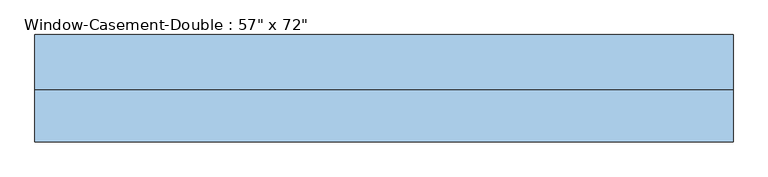
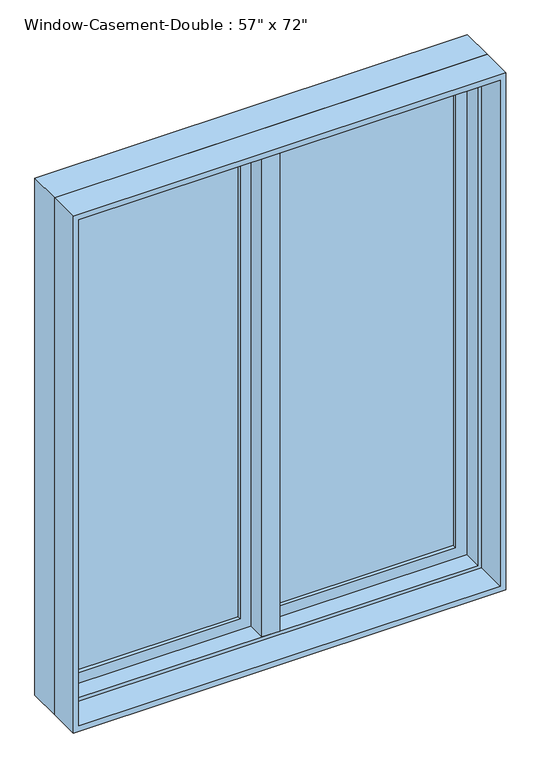
"""IFC4 building model written with IfcOpenShell, lengths in millimetres: window geometry."""

from ifc_helpers import new_model, si_unit, frame, origin, place, context, project, spatial, polyline, outline, extrude, faceted_brep, source, transform, mapped, element, save


def window_c580ef63(model_context):
    return source(origin(), model_context, "Body", "SolidModel", [
        faceted_brep([(9.525, 120.65, 2730.5), (-9.525, 120.65, 2730.5), (-9.525, 69.85, 2730.5), (9.525, 69.85, 2730.5), (9.525, 120.65, 927.1), (9.525, 69.85, 927.1), (-9.525, 69.85, 927.1), (-9.525, 120.65, 927.1), (-9.525, 69.85, 946.15), (-9.525, 69.85, 2711.45), (-30.1625, 69.85, 946.15), (-30.1625, 69.85, 2711.45), (-30.1625, 6.35, 946.15), (-30.1625, 6.35, 2711.45), (30.1625, 6.35, 946.15), (30.1625, 6.35, 2711.45), (30.1625, 69.85, 946.15), (30.1625, 69.85, 2711.45), (9.525, 69.85, 946.15), (9.525, 69.85, 2711.45)], [[[0, 1, 2, 3]], [[4, 5, 6, 7]], [[1, 0, 4, 7]], [[2, 1, 7, 6, 8, 9]], [[9, 8, 10, 11]], [[11, 10, 12, 13]], [[13, 12, 14, 15]], [[15, 14, 16, 17]], [[17, 16, 18, 19]], [[0, 3, 19, 18, 5, 4]], [[18, 8, 6, 5]], [[9, 19, 3, 2]], [[8, 18, 16, 14, 12, 10]], [[19, 9, 11, 13, 15, 17]]]),
        extrude(outline(polyline([(-66.675, 101.6), (-66.675, 95.25), (-654.05, 95.25), (-654.05, 101.6), (-66.675, 101.6)])), frame((0.0, 0.0, 984.25), z_axis=(0.0, 0.0, 1.0), x_axis=(1.0, 0.0, 0.0)), (0.0, 0.0, 1.0), 1689.1),
        extrude(outline(polyline([(-654.05, 82.55), (-654.05, 88.9), (-66.675, 88.9), (-66.675, 82.55), (-654.05, 82.55)])), frame((0.0, 0.0, 984.25), z_axis=(0.0, 0.0, 1.0), x_axis=(1.0, 0.0, 0.0)), (0.0, 0.0, 1.0), 1689.1),
        extrude(outline(polyline([(654.05, 101.6), (654.05, 95.25), (66.675, 95.25), (66.675, 101.6), (654.05, 101.6)])), frame((0.0, 0.0, 984.25), z_axis=(0.0, 0.0, 1.0), x_axis=(1.0, 0.0, 0.0)), (0.0, 0.0, 1.0), 1689.1),
        extrude(outline(polyline([(66.675, 82.55), (66.675, 88.9), (654.05, 88.9), (654.05, 82.55), (66.675, 82.55)])), frame((0.0, 0.0, 984.25), z_axis=(0.0, 0.0, 1.0), x_axis=(1.0, 0.0, 0.0)), (0.0, 0.0, 1.0), 1689.1),
        extrude(outline(polyline([(2730.5, -711.2), (927.1, -711.2), (927.1, -9.525), (2730.5, -9.525), (2730.5, -711.2)]), holes=[polyline([(2673.35, -66.675), (984.25, -66.675), (984.25, -654.05), (2673.35, -654.05), (2673.35, -66.675)])]), frame((0.0, 69.85, 0.0), z_axis=(0.0, 1.0, 0.0), x_axis=(0.0, 0.0, 1.0)), (0.0, 0.0, 1.0), 44.45),
        extrude(outline(polyline([(927.1, 711.2), (2730.5, 711.2), (2730.5, 9.525), (927.1, 9.525), (927.1, 711.2)]), holes=[polyline([(984.25, 66.675), (2673.35, 66.675), (2673.35, 654.05), (984.25, 654.05), (984.25, 66.675)])]), frame((0.0, 69.85, 0.0), z_axis=(0.0, 1.0, 0.0), x_axis=(0.0, 0.0, 1.0)), (0.0, 0.0, 1.0), 44.45),
        extrude(outline(polyline([(2743.2, -723.9), (914.4, -723.9), (914.4, 723.9), (2743.2, 723.9), (2743.2, -723.9)]), holes=[polyline([(2724.15, 704.85), (933.45, 704.85), (933.45, -704.85), (2724.15, -704.85), (2724.15, 704.85)])]), frame((0.0, -101.6, 0.0), z_axis=(0.0, 1.0, 0.0), x_axis=(0.0, 0.0, 1.0)), (0.0, 0.0, 1.0), 107.95),
        faceted_brep([(692.15, 69.85, 2711.45), (692.15, 6.35, 2711.45), (-692.15, 6.35, 2711.45), (-692.15, 69.85, 2711.45), (711.2, 120.65, 2730.5), (711.2, 69.85, 2730.5), (-711.2, 69.85, 2730.5), (-711.2, 120.65, 2730.5), (723.9, 6.35, 2743.2), (723.9, 120.65, 2743.2), (-723.9, 120.65, 2743.2), (-723.9, 6.35, 2743.2), (-692.15, 6.35, 946.15), (-692.15, 69.85, 946.15), (-711.2, 69.85, 927.1), (-711.2, 120.65, 927.1), (-723.9, 120.65, 914.4), (-723.9, 6.35, 914.4), (692.15, 6.35, 946.15), (692.15, 69.85, 946.15), (711.2, 69.85, 927.1), (711.2, 120.65, 927.1), (723.9, 120.65, 914.4), (723.9, 6.35, 914.4)], [[[0, 1, 2, 3]], [[4, 5, 6, 7]], [[8, 9, 10, 11]], [[3, 2, 12, 13]], [[7, 6, 14, 15]], [[11, 10, 16, 17]], [[13, 12, 18, 19]], [[15, 14, 20, 21]], [[17, 16, 22, 23]], [[11, 17, 23, 8], [1, 18, 12, 2]], [[19, 18, 1, 0]], [[5, 20, 14, 6], [3, 13, 19, 0]], [[21, 20, 5, 4]], [[23, 22, 9, 8]], [[9, 22, 16, 10], [7, 15, 21, 4]]]),
    ])


if __name__ == "__main__":
    model = new_model("IFC4")
    model_context = context("Model", 3, world=origin())
    ifc_project = project(units=[si_unit("LENGTHUNIT", "METRE", prefix="MILLI")], contexts=[model_context])
    site = spatial("IfcSite", under=ifc_project)
    building = spatial("IfcBuilding", under=site)
    placement = place(None, origin())
    window_shape = window_c580ef63(model_context)
    element("IfcWindow", 1, ObjectType="Window-Casement-Double : 57\" x 72\"", at=placement, inside=building, context=model_context, shape_type="MappedRepresentation", body=[
        mapped(window_shape, transform((0.0, 0.0, 0.0), x_axis=(1.0, 0.0, 0.0), y_axis=(0.0, 1.0, 0.0), z_axis=(0.0, 0.0, 1.0))),
    ])
    save(model, "model.ifc")

# Revit data of these elements
# Type "Window-Casement-Double : 57\" x 72\""
#   Type Mark = "62"
#   Fire Rating = "0.5h"
#   Assembly Code = "B2020100"
#   Analytic Construction = "Double glazing - domestic"
#   Frame Extension [instance default] = 0' - 0 1/4"
#   Window Inset [instance default] = 0' - 0"
#   Wall Thickness [instance default] = 0' - 6"
#   Interior Wall Closure [instance default] = 0' - 2 1/4"
#   Half Width = 2' - 4 1/2"
#   Visual Light Transmittance = 0.81
#   Thermal Resistance (R) = 1.8146 (h·ft²·°F)/BTU
#   Solar Heat Gain Coefficient = 0.76
#   Rough Width = 4' - 9 1/2"
#   Rough Height = 6' - 0 1/2"
#   Height = 6' - 0"
#   Heat Transfer Coefficient (U) = 0.5511 BTU/(h·ft²·°F)
#   Exterior Wall Closure [instance default] = 0' - 1 1/4"
#   Extension Jamb [instance default] = 0' - 2 1/4"
#   Default Sill Height = 3' - 0"
#   Width = 4' - 9"
#   Define Thermal Properties by = 0
#   Muntin Visibility = yes
#   Interior Trim Visibility [instance default] = yes
#   Exterior Trim Visibility [instance default] = yes
#   Extension Jamb Visibility [instance default] = yes
#   Interior Trim Material = Wood - Stained
#   Muntin Pattern = Muntin Pattern_2x2 : Muntin Pattern_2x2
#   Interior Trim = Trim-Window-Interior-Flat : Picture Frame
#   Interior Frame Material = Wood - Stained
#   Glass Panel Material = Glass
#   Exterior Trim Material = Clad - White
#   Exterior Trim = Trim-Window-Exterior-Flat : with Sill
#   Exterior Frame Material = Clad - White
#   Wall Closure = (empty or 0)
# Element 1 (IfcWindow, "Window-Casement-Double : 57\" x 72\"")
#   Wall Thickness = 0' - 8"
#   Extension Jamb = 0' - 4 1/4"
#   Materials on its faces: "Wood - Stained", "Glass", "Clad - White"
# Materials
#   "Wood - Stained": class "Wood", colour RGB 224 178 126, transparency 0, Cost = 0
#   "Glass": class "Glass", colour RGB 236 240 239, transparency 0.5, Description = "Soda Lime Glass", Cost = 0
#   "Clad - White": class "Wood", colour RGB 216 216 204, transparency 0, Cost = 0
